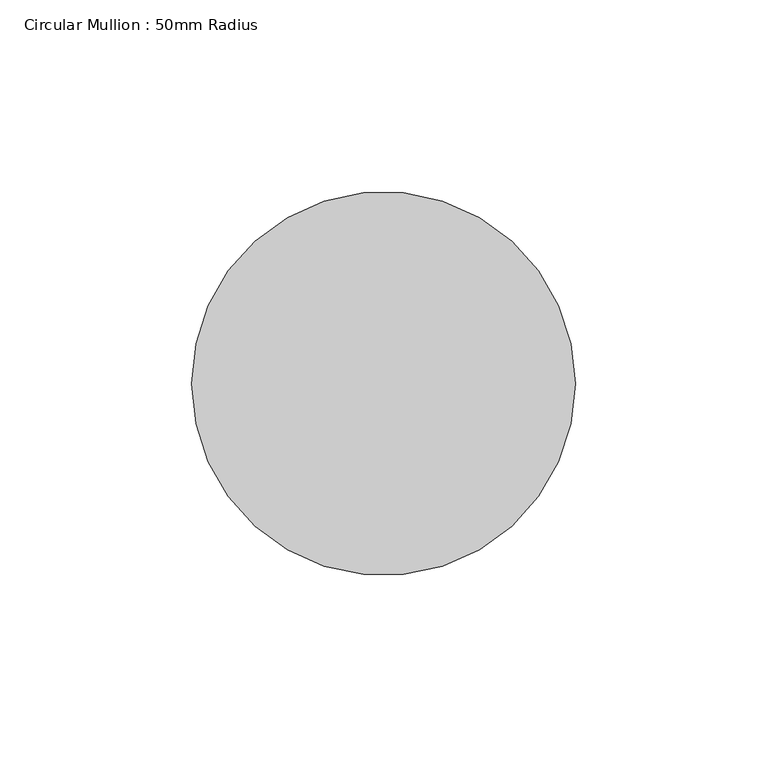
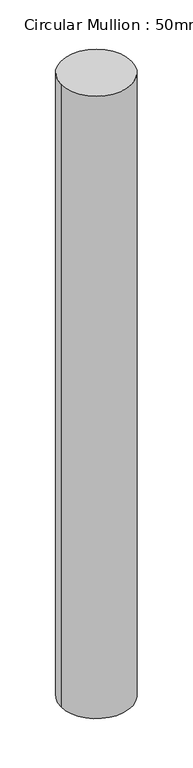
"""IFC4 building model written with IfcOpenShell, lengths in millimetres: member geometry, Circular Mullion : 50mm Radius."""

from ifc_helpers import new_model, si_unit, point, frame, origin, origin_2d, place, context, project, spatial, circle_curve, trimmed, segment, composite_curve, outline, extrude, source, transform, mapped, element, save


def circular_mullion_50mm_radius_ce57bd47(model_context):
    return source(origin(), model_context, "Body", "SweptSolid", [
        extrude(outline(composite_curve([segment(trimmed(circle_curve(origin_2d(), 50.0), [point((50.0, 0.0))], [point((-50.0, 0.0))], False, "CARTESIAN"), True, "CONTINUOUS"), segment(trimmed(circle_curve(origin_2d(), 50.0), [point((-50.0, 0.0))], [point((50.0, 0.0))], False, "CARTESIAN"), True, "CONTINUOUS")], self_intersect=False)), frame((0.0, 0.0, -931.3242969), z_axis=(0.0, 0.0, 1.0), x_axis=(1.0, 0.0, 0.0)), (0.0, 0.0, 1.0), 931.3242969),
    ])


if __name__ == "__main__":
    model = new_model("IFC4")
    model_context = context("Model", 3, world=origin())
    ifc_project = project(units=[si_unit("LENGTHUNIT", "METRE", prefix="MILLI")], contexts=[model_context])
    site = spatial("IfcSite", under=ifc_project)
    building = spatial("IfcBuilding", under=site)
    placement = place(None, origin())
    circular_mullion_50mm_radius_shape = circular_mullion_50mm_radius_ce57bd47(model_context)
    element("IfcMember", 1, ObjectType="Circular Mullion : 50mm Radius", at=placement, inside=building, context=model_context, shape_type="MappedRepresentation", body=[
        mapped(circular_mullion_50mm_radius_shape, transform((0.0, 0.0, 0.0), x_axis=(1.0, 0.0, 0.0), y_axis=(0.0, 1.0, 0.0), z_axis=(0.0, 0.0, 1.0))),
    ])
    save(model, "model.ifc")

# Revit data of these elements
# Type "Circular Mullion : 50mm Radius"
#   built-in parameter 1007350 = 0.164042 (stored number, unit not read)
# Element 1 (IfcMember, "Circular Mullion : 50mm Radius")
#   Materials on its faces: "Aluminium"
# Materials
#   "Aluminium": class "Metal", colour RGB 247 247 247, transparency 0, Description = "Aluminium 6061", Cost = 0
